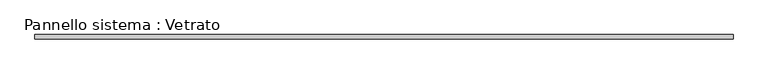
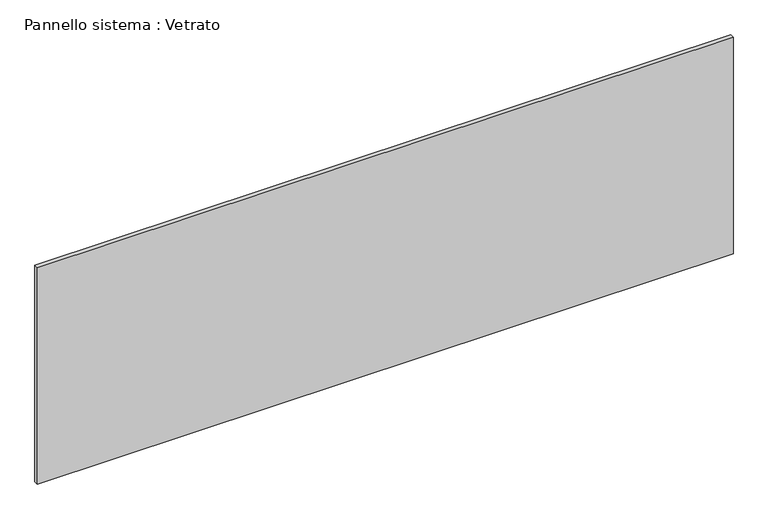
"""IFC4 building model written with IfcOpenShell, lengths in millimetres: plate geometry, Pannello sistema : Vetrato."""

from ifc_helpers import new_model, si_unit, origin, origin_with_axes, place, context, project, spatial, polyline, outline, extrude, source, transform, mapped, element, save


def pannello_sistema_vetrato_c31b63d1(model_context):
    return source(origin(), model_context, "Body", "SweptSolid", [
        extrude(outline(polyline([(2502.5, -15.0), (-2502.5, -15.0), (-2502.5, 15.0), (2502.5, 15.0), (2502.5, -15.0)])), origin_with_axes(), (0.0, 0.0, 1.0), 1645.0),
    ])


if __name__ == "__main__":
    model = new_model("IFC4")
    model_context = context("Model", 3, world=origin())
    ifc_project = project(units=[si_unit("LENGTHUNIT", "METRE", prefix="MILLI")], contexts=[model_context])
    site = spatial("IfcSite", under=ifc_project)
    building = spatial("IfcBuilding", under=site)
    placement = place(None, origin())
    pannello_sistema_vetrato_shape = pannello_sistema_vetrato_c31b63d1(model_context)
    element("IfcPlate", 1, ObjectType="Pannello sistema : Vetrato", at=placement, inside=building, context=model_context, shape_type="MappedRepresentation", body=[
        mapped(pannello_sistema_vetrato_shape, transform((0.0, 0.0, 0.0), x_axis=(1.0, 0.0, 0.0), y_axis=(0.0, 1.0, 0.0), z_axis=(0.0, 0.0, 1.0))),
    ])
    save(model, "model.ifc")

# Revit data of these elements
# Type "Pannello sistema : Vetrato"
#   Construction Type Id = "GSP4R"
#   Analytic Construction = "Vetrata singola Pilkington 1/8 in"
#   Visual Light Transmittance = 0.9
#   Solar Heat Gain Coefficient = 0.86
#   Heat Transfer Coefficient (U) = 6.7069 W/(m²·K)
# Element 1 (IfcPlate, "Pannello sistema : Vetrato")
#   Materials on its faces: "Default - Vetro"
# Materials
#   "Default - Vetro": class "Vetro", colour RGB 208 208 208, transparency 0.7, Cost = 0
